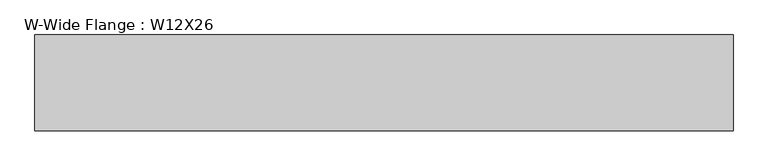
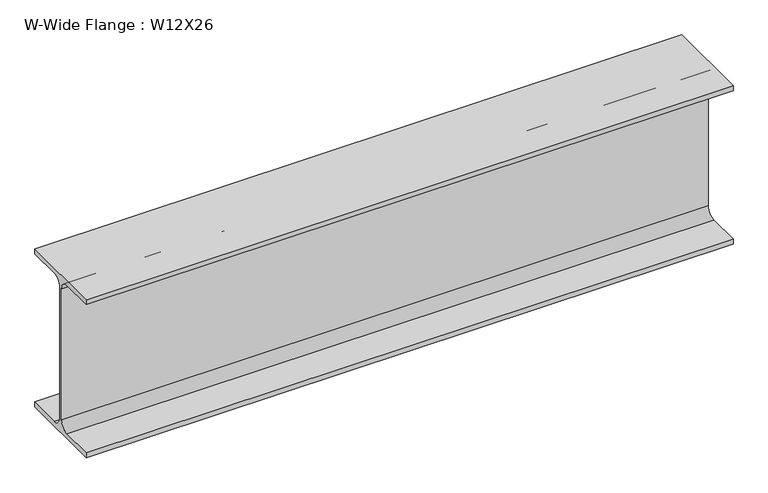
"""IFC4 building model written with IfcOpenShell, lengths in millimetres: beam geometry, W-Wide Flange : W12X26."""

import ifcopenshell
import ifcopenshell.guid

model = None  # the IFC model being written
_history = None  # IfcOwnerHistory: only IFC2X3 demands one
_inside = {}  # id of a spatial element -> (the spatial element, [elements in it])
_under = {}  # id of a project, library or spatial element -> (it, [spatial elements below it])
_declared = {}  # id of a project -> (the project, [libraries it declares])
_typed = {}  # id of a type object -> (the type object, [elements of that type])
_made_of = {}  # id of a material, layer set ... -> (it, [elements and type objects made of it])


def new_model(schema):
    """Start an empty IFC model of exactly this schema.

    Asked for "IFC4X3", IfcOpenShell would pick the latest addendum, in which some entities
    have other attributes; the version numbers below select the first issue.
    IFC2X3 requires an IfcOwnerHistory on every rooted entity: one is made here for all.
    """
    global model, _history
    if schema == "IFC4X3":
        model = ifcopenshell.file(schema_version=(4, 3, 0, 0))
    else:
        model = ifcopenshell.file(schema=schema)
    _inside.clear()
    _under.clear()
    _declared.clear()
    _typed.clear()
    _made_of.clear()
    _history = None
    if model.schema == "IFC2X3":
        org = make("IfcOrganization", Name="unknown")
        user = make(
            "IfcPersonAndOrganization",
            ThePerson=make("IfcPerson", FamilyName="unknown"),
            TheOrganization=org,
        )
        app = make(
            "IfcApplication",
            ApplicationDeveloper=org,
            Version="unknown",
            ApplicationFullName="unknown",
            ApplicationIdentifier="unknown",
        )
        _history = make(
            "IfcOwnerHistory",
            OwningUser=user,
            OwningApplication=app,
            ChangeAction="ADDED",
            CreationDate=0,
        )
    return model


def make(cls, **values):
    """One entity of the class cls with the attributes given. An attribute that is None is left unset."""
    return model.create_entity(
        cls, **{name: value for name, value in values.items() if value is not None}
    )


def rooted(cls, **values):
    """An entity with a GlobalId (a new one), such as an element, a storey or a relation."""
    return make(cls, GlobalId=ifcopenshell.guid.new(), OwnerHistory=_history, **values)


def si_unit(unit_type, name, prefix=None):
    """IfcSIUnit, for example si_unit("LENGTHUNIT", "METRE", prefix="MILLI")."""
    return make("IfcSIUnit", UnitType=unit_type, Prefix=prefix, Name=name)


def assignment(units):
    """IfcUnitAssignment: the units of a project."""
    return None if units is None else make("IfcUnitAssignment", Units=units)


def point(xyz):
    """IfcCartesianPoint."""
    return None if xyz is None else make("IfcCartesianPoint", Coordinates=xyz)


def direction(xyz):
    """IfcDirection."""
    return None if xyz is None else make("IfcDirection", DirectionRatios=xyz)


def frame(location, z_axis=None, x_axis=None):
    """IfcAxis2Placement3D, a coordinate frame: its origin and axes. An axis left out is left unset."""
    return make(
        "IfcAxis2Placement3D",
        Location=point(location),
        Axis=direction(z_axis),
        RefDirection=direction(x_axis),
    )


def frame_2d(location, x_axis=None):
    """IfcAxis2Placement2D, a coordinate frame in the plane: its origin and x axis."""
    return make(
        "IfcAxis2Placement2D", Location=point(location), RefDirection=direction(x_axis)
    )


def origin():
    """The frame at (0, 0, 0) with its axes left unset."""
    return frame((0.0, 0.0, 0.0))


def place(relative_to, where):
    """IfcLocalPlacement: puts the frame where relative to a parent placement (None: the world)."""
    return make(
        "IfcLocalPlacement", PlacementRelTo=relative_to, RelativePlacement=where
    )


def context(
    kind, dimensions, precision=None, world=None, true_north=None, identifier=None
):
    """IfcGeometricRepresentationContext, for example the 3D "Model" context."""
    return make(
        "IfcGeometricRepresentationContext",
        ContextIdentifier=identifier,
        ContextType=kind,
        CoordinateSpaceDimension=dimensions,
        Precision=precision,
        WorldCoordinateSystem=world,
        TrueNorth=true_north,
    )


def project(units=None, contexts=None):
    """IfcProject with its units and contexts."""
    return rooted(
        "IfcProject",
        Name="project",
        RepresentationContexts=contexts,
        UnitsInContext=assignment(units),
    )


def spatial(cls, under=None, at=None, **own):
    """A site, building, storey or space (cls), placed at a placement, below another one or the project."""
    s = rooted(cls, ObjectPlacement=at, **own)
    if under is not None:
        _under.setdefault(under.id(), (under, []))[1].append(s)
    return s


def polyline(points):
    """IfcPolyline through the points."""
    return make("IfcPolyline", Points=[point(p) for p in points])


def circle_curve(where, radius):
    """IfcCircle in the frame where."""
    return make("IfcCircle", Position=where, Radius=radius)


def trimmed(basis, trim1, trim2, sense, master):
    """IfcTrimmedCurve: the piece of a basis curve between two trims."""
    return make(
        "IfcTrimmedCurve",
        BasisCurve=basis,
        Trim1=trim1,
        Trim2=trim2,
        SenseAgreement=sense,
        MasterRepresentation=master,
    )


def segment(curve, same_sense, transition):
    """IfcCompositeCurveSegment."""
    return make(
        "IfcCompositeCurveSegment",
        Transition=transition,
        SameSense=same_sense,
        ParentCurve=curve,
    )


def composite_curve(segments, self_intersect=None):
    """IfcCompositeCurve: segments joined end to end."""
    return make("IfcCompositeCurve", Segments=segments, SelfIntersect=self_intersect)


def outline(outer, holes=None, kind="AREA"):
    """IfcArbitraryClosedProfileDef: a profile drawn as a closed curve; with holes, ...WithVoids."""
    if holes is None:
        return make("IfcArbitraryClosedProfileDef", ProfileType=kind, OuterCurve=outer)
    return make(
        "IfcArbitraryProfileDefWithVoids",
        ProfileType=kind,
        OuterCurve=outer,
        InnerCurves=holes,
    )


def extrude(swept, where, along, depth):
    """IfcExtrudedAreaSolid: the profile swept, set in the frame where, extruded along a direction by depth."""
    return make(
        "IfcExtrudedAreaSolid",
        SweptArea=swept,
        Position=where,
        ExtrudedDirection=direction(along),
        Depth=depth,
    )


def shape(context_of_items, identifier, shape_type, items):
    """IfcShapeRepresentation: the items that make up one representation, for example the "Body"."""
    return make(
        "IfcShapeRepresentation",
        ContextOfItems=context_of_items,
        RepresentationIdentifier=identifier,
        RepresentationType=shape_type,
        Items=items,
    )


def source(mapping_origin, context_of_items, identifier, shape_type, items):
    """IfcRepresentationMap: a shape defined once, which mapped items show again and again."""
    return make(
        "IfcRepresentationMap",
        MappingOrigin=mapping_origin,
        MappedRepresentation=shape(context_of_items, identifier, shape_type, items),
    )


def transform(
    local_origin,
    x_axis=None,
    y_axis=None,
    z_axis=None,
    scale=None,
    scale2=None,
    scale3=None,
    uniform=True,
):
    """IfcCartesianTransformationOperator3D, or its non-uniform kind. x_axis, y_axis, z_axis: its Axis1, 2, 3."""
    if uniform:
        return make(
            "IfcCartesianTransformationOperator3D",
            Axis1=direction(x_axis),
            Axis2=direction(y_axis),
            LocalOrigin=point(local_origin),
            Scale=scale,
            Axis3=direction(z_axis),
        )
    return make(
        "IfcCartesianTransformationOperator3DnonUniform",
        Axis1=direction(x_axis),
        Axis2=direction(y_axis),
        LocalOrigin=point(local_origin),
        Scale=scale,
        Axis3=direction(z_axis),
        Scale2=scale2,
        Scale3=scale3,
    )


def mapped(mapping_source, mapping_target):
    """IfcMappedItem: shows the shape of a source again, moved by a transform."""
    return make(
        "IfcMappedItem", MappingSource=mapping_source, MappingTarget=mapping_target
    )


def made_of(thing, what):
    """Note that an element or type object is made of a material, layer set ...; save() writes the relation."""
    if what is not None:
        _made_of.setdefault(what.id(), (what, []))[1].append(thing)
    return thing


def element(
    cls,
    number,
    at=None,
    inside=None,
    cuts=None,
    type_object=None,
    material=None,
    context=None,
    identifier="Body",
    shape_type=None,
    held_by="IfcProductDefinitionShape",
    body=None,
    shapes=None,
    **own,
):
    """One element of the class cls, such as IfcWall. Its Tag is "e" and its number.

    at: its placement. inside: the storey or other place that contains it. cuts: it is an
    opening in that element (IfcRelVoidsElement). A single representation is given by context,
    identifier, shape_type and body (its items); several are given by shapes. held_by: the class
    of the entity that holds the representations. save() writes the other relations.
    """
    e = rooted(cls, Tag="e%d" % number, ObjectPlacement=at, **own)
    if body is not None:
        shapes = [shape(context, identifier, shape_type, body)]
    if shapes is not None:
        e.Representation = make(held_by, Representations=shapes)
    if inside is not None:
        _inside.setdefault(inside.id(), (inside, []))[1].append(e)
    if cuts is not None:
        rooted(
            "IfcRelVoidsElement", RelatingBuildingElement=cuts, RelatedOpeningElement=e
        )
    if type_object is not None:
        _typed.setdefault(type_object.id(), (type_object, []))[1].append(e)
    return made_of(e, material)


def aggregate(whole, parts):
    """IfcRelAggregates: a whole, such as a stair, and the parts it consists of."""
    return rooted("IfcRelAggregates", RelatingObject=whole, RelatedObjects=parts)


def save(model, path):
    """Write the relations noted so far, then the file.

    IfcRelAggregates (storeys below a building ...), IfcRelContainedInSpatialStructure (elements
    in a storey), IfcRelDefinesByType, IfcRelAssociatesMaterial and IfcRelDeclares: one each for
    every whole, place, type object, material and project.
    """
    for whole, parts in _under.values():
        aggregate(whole, parts)
    for where, things in _inside.values():
        rooted(
            "IfcRelContainedInSpatialStructure",
            RelatedElements=things,
            RelatingStructure=where,
        )
    for kind, things in _typed.values():
        rooted("IfcRelDefinesByType", RelatedObjects=things, RelatingType=kind)
    for what, things in _made_of.values():
        rooted("IfcRelAssociatesMaterial", RelatedObjects=things, RelatingMaterial=what)
    for by, libraries in _declared.values():
        rooted("IfcRelDeclares", RelatingContext=by, RelatedDefinitions=libraries)
    model.write(path)


def w_wide_flange_w12x26_8f29fc3b(model_context):
    return source(origin(), model_context, "Body", "SweptSolid", [
        extrude(outline(composite_curve([segment(polyline([(82.4011719, -145.5539063), (82.4011719, -155.178125), (-82.4011719, -155.178125), (-82.4011719, -145.5539063), (-20.2902344, -145.5539063)]), True, "CONTINUOUS"), segment(trimmed(circle_curve(frame_2d((-20.2902344, -128.190625)), 17.3632812), [point((-20.2902344, -145.5539063))], [point((-2.9269531, -128.190625))], True, "CARTESIAN"), True, "CONTINUOUS"), segment(polyline([(-2.9269531, -128.190625), (-2.9269531, 128.190625)]), True, "CONTINUOUS"), segment(trimmed(circle_curve(frame_2d((-20.2902344, 128.190625)), 17.3632812), [point((-2.9269531, 128.190625))], [point((-20.2902344, 145.5539062))], True, "CARTESIAN"), True, "CONTINUOUS"), segment(polyline([(-20.2902344, 145.5539062), (-82.4011719, 145.5539062), (-82.4011719, 155.178125), (82.4011719, 155.178125), (82.4011719, 145.5539062), (20.2902344, 145.5539062)]), True, "CONTINUOUS"), segment(trimmed(circle_curve(frame_2d((20.2902344, 128.190625)), 17.3632812), [point((20.2902344, 145.5539062))], [point((2.9269531, 128.190625))], True, "CARTESIAN"), True, "CONTINUOUS"), segment(polyline([(2.9269531, 128.190625), (2.9269531, -128.190625)]), True, "CONTINUOUS"), segment(trimmed(circle_curve(frame_2d((20.2902344, -128.190625)), 17.3632812), [point((2.9269531, -128.190625))], [point((20.2902344, -145.5539063))], True, "CARTESIAN"), True, "CONTINUOUS"), segment(polyline([(20.2902344, -145.5539063), (82.4011719, -145.5539063)]), True, "CONTINUOUS")], self_intersect=False)), frame((-641.2011719, 0.0, 0.0), z_axis=(1.0, 0.0, 0.0), x_axis=(0.0, 1.0, 0.0)), (0.0, 0.0, 1.0), 1200.0011719),
    ])


if __name__ == "__main__":
    model = new_model("IFC4")
    model_context = context("Model", 3, world=origin())
    ifc_project = project(units=[si_unit("LENGTHUNIT", "METRE", prefix="MILLI")], contexts=[model_context])
    site = spatial("IfcSite", under=ifc_project)
    building = spatial("IfcBuilding", under=site)
    placement = place(None, origin())
    w_wide_flange_w12x26_shape = w_wide_flange_w12x26_8f29fc3b(model_context)
    element("IfcBeam", 1, ObjectType="W-Wide Flange : W12X26", at=placement, inside=building, context=model_context, shape_type="MappedRepresentation", body=[
        mapped(w_wide_flange_w12x26_shape, transform((0.0, 0.0, 0.0), x_axis=(1.0, 0.0, 0.0), y_axis=(0.0, 1.0, 0.0), z_axis=(0.0, 0.0, 1.0))),
    ])
    save(model, "model.ifc")

# Revit data of these elements
# Type "W-Wide Flange : W12X26"
#   Assembly Code = "B10"
#   W = 26
#   Length [instance default] = 5' - 0"
#   bf = 0' - 6 125/256"
#   d = 1' - 0 7/32"
#   k = 0' - 1 1/16"
#   k2 = 0' - 0 175/256"
#   tf = 0' - 0 97/256"
#   tw = 0' - 0 59/256"
#   A = 0.053125 SF
#   Structural Material [instance default] = none
# Element 1 (IfcBeam, "W-Wide Flange : W12X26")
#   Structural Material = Dark metal
#   Materials on its faces: "Dark metal"
# Materials
#   "Dark metal": class "Generic", colour RGB 44 29 29, transparency 0, Cost = 0
